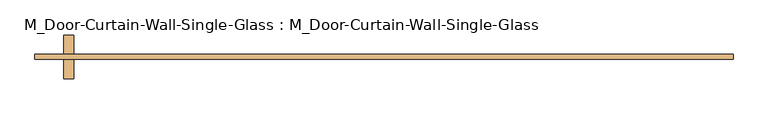
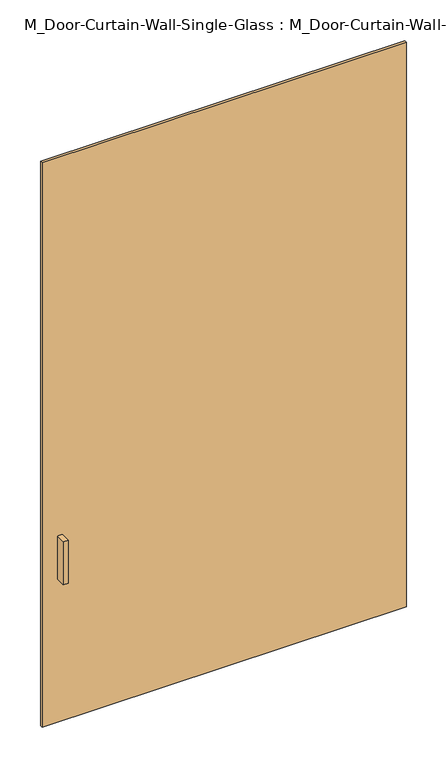
"""IFC4 building model written with IfcOpenShell, lengths in millimetres: door geometry, M_Door-Curtain-Wall-Single-Glass : M_Door-Curtain-Wall-Single-Glass."""

import ifcopenshell
import ifcopenshell.guid

model = None  # the IFC model being written
_history = None  # IfcOwnerHistory: only IFC2X3 demands one
_inside = {}  # id of a spatial element -> (the spatial element, [elements in it])
_under = {}  # id of a project, library or spatial element -> (it, [spatial elements below it])
_declared = {}  # id of a project -> (the project, [libraries it declares])
_typed = {}  # id of a type object -> (the type object, [elements of that type])
_made_of = {}  # id of a material, layer set ... -> (it, [elements and type objects made of it])


def new_model(schema):
    """Start an empty IFC model of exactly this schema.

    Asked for "IFC4X3", IfcOpenShell would pick the latest addendum, in which some entities
    have other attributes; the version numbers below select the first issue.
    IFC2X3 requires an IfcOwnerHistory on every rooted entity: one is made here for all.
    """
    global model, _history
    if schema == "IFC4X3":
        model = ifcopenshell.file(schema_version=(4, 3, 0, 0))
    else:
        model = ifcopenshell.file(schema=schema)
    _inside.clear()
    _under.clear()
    _declared.clear()
    _typed.clear()
    _made_of.clear()
    _history = None
    if model.schema == "IFC2X3":
        org = make("IfcOrganization", Name="unknown")
        user = make(
            "IfcPersonAndOrganization",
            ThePerson=make("IfcPerson", FamilyName="unknown"),
            TheOrganization=org,
        )
        app = make(
            "IfcApplication",
            ApplicationDeveloper=org,
            Version="unknown",
            ApplicationFullName="unknown",
            ApplicationIdentifier="unknown",
        )
        _history = make(
            "IfcOwnerHistory",
            OwningUser=user,
            OwningApplication=app,
            ChangeAction="ADDED",
            CreationDate=0,
        )
    return model


def make(cls, **values):
    """One entity of the class cls with the attributes given. An attribute that is None is left unset."""
    return model.create_entity(
        cls, **{name: value for name, value in values.items() if value is not None}
    )


def rooted(cls, **values):
    """An entity with a GlobalId (a new one), such as an element, a storey or a relation."""
    return make(cls, GlobalId=ifcopenshell.guid.new(), OwnerHistory=_history, **values)


def si_unit(unit_type, name, prefix=None):
    """IfcSIUnit, for example si_unit("LENGTHUNIT", "METRE", prefix="MILLI")."""
    return make("IfcSIUnit", UnitType=unit_type, Prefix=prefix, Name=name)


def assignment(units):
    """IfcUnitAssignment: the units of a project."""
    return None if units is None else make("IfcUnitAssignment", Units=units)


def point(xyz):
    """IfcCartesianPoint."""
    return None if xyz is None else make("IfcCartesianPoint", Coordinates=xyz)


def direction(xyz):
    """IfcDirection."""
    return None if xyz is None else make("IfcDirection", DirectionRatios=xyz)


def frame(location, z_axis=None, x_axis=None):
    """IfcAxis2Placement3D, a coordinate frame: its origin and axes. An axis left out is left unset."""
    return make(
        "IfcAxis2Placement3D",
        Location=point(location),
        Axis=direction(z_axis),
        RefDirection=direction(x_axis),
    )


def origin():
    """The frame at (0, 0, 0) with its axes left unset."""
    return frame((0.0, 0.0, 0.0))


def origin_with_axes():
    """The frame at (0, 0, 0) with the z axis (0, 0, 1) and the x axis (1, 0, 0) written out."""
    return frame((0.0, 0.0, 0.0), z_axis=(0.0, 0.0, 1.0), x_axis=(1.0, 0.0, 0.0))


def place(relative_to, where):
    """IfcLocalPlacement: puts the frame where relative to a parent placement (None: the world)."""
    return make(
        "IfcLocalPlacement", PlacementRelTo=relative_to, RelativePlacement=where
    )


def context(
    kind, dimensions, precision=None, world=None, true_north=None, identifier=None
):
    """IfcGeometricRepresentationContext, for example the 3D "Model" context."""
    return make(
        "IfcGeometricRepresentationContext",
        ContextIdentifier=identifier,
        ContextType=kind,
        CoordinateSpaceDimension=dimensions,
        Precision=precision,
        WorldCoordinateSystem=world,
        TrueNorth=true_north,
    )


def project(units=None, contexts=None):
    """IfcProject with its units and contexts."""
    return rooted(
        "IfcProject",
        Name="project",
        RepresentationContexts=contexts,
        UnitsInContext=assignment(units),
    )


def spatial(cls, under=None, at=None, **own):
    """A site, building, storey or space (cls), placed at a placement, below another one or the project."""
    s = rooted(cls, ObjectPlacement=at, **own)
    if under is not None:
        _under.setdefault(under.id(), (under, []))[1].append(s)
    return s


def polyline(points):
    """IfcPolyline through the points."""
    return make("IfcPolyline", Points=[point(p) for p in points])


def outline(outer, holes=None, kind="AREA"):
    """IfcArbitraryClosedProfileDef: a profile drawn as a closed curve; with holes, ...WithVoids."""
    if holes is None:
        return make("IfcArbitraryClosedProfileDef", ProfileType=kind, OuterCurve=outer)
    return make(
        "IfcArbitraryProfileDefWithVoids",
        ProfileType=kind,
        OuterCurve=outer,
        InnerCurves=holes,
    )


def extrude(swept, where, along, depth):
    """IfcExtrudedAreaSolid: the profile swept, set in the frame where, extruded along a direction by depth."""
    return make(
        "IfcExtrudedAreaSolid",
        SweptArea=swept,
        Position=where,
        ExtrudedDirection=direction(along),
        Depth=depth,
    )


def shape(context_of_items, identifier, shape_type, items):
    """IfcShapeRepresentation: the items that make up one representation, for example the "Body"."""
    return make(
        "IfcShapeRepresentation",
        ContextOfItems=context_of_items,
        RepresentationIdentifier=identifier,
        RepresentationType=shape_type,
        Items=items,
    )


def source(mapping_origin, context_of_items, identifier, shape_type, items):
    """IfcRepresentationMap: a shape defined once, which mapped items show again and again."""
    return make(
        "IfcRepresentationMap",
        MappingOrigin=mapping_origin,
        MappedRepresentation=shape(context_of_items, identifier, shape_type, items),
    )


def transform(
    local_origin,
    x_axis=None,
    y_axis=None,
    z_axis=None,
    scale=None,
    scale2=None,
    scale3=None,
    uniform=True,
):
    """IfcCartesianTransformationOperator3D, or its non-uniform kind. x_axis, y_axis, z_axis: its Axis1, 2, 3."""
    if uniform:
        return make(
            "IfcCartesianTransformationOperator3D",
            Axis1=direction(x_axis),
            Axis2=direction(y_axis),
            LocalOrigin=point(local_origin),
            Scale=scale,
            Axis3=direction(z_axis),
        )
    return make(
        "IfcCartesianTransformationOperator3DnonUniform",
        Axis1=direction(x_axis),
        Axis2=direction(y_axis),
        LocalOrigin=point(local_origin),
        Scale=scale,
        Axis3=direction(z_axis),
        Scale2=scale2,
        Scale3=scale3,
    )


def mapped(mapping_source, mapping_target):
    """IfcMappedItem: shows the shape of a source again, moved by a transform."""
    return make(
        "IfcMappedItem", MappingSource=mapping_source, MappingTarget=mapping_target
    )


def made_of(thing, what):
    """Note that an element or type object is made of a material, layer set ...; save() writes the relation."""
    if what is not None:
        _made_of.setdefault(what.id(), (what, []))[1].append(thing)
    return thing


def element(
    cls,
    number,
    at=None,
    inside=None,
    cuts=None,
    type_object=None,
    material=None,
    context=None,
    identifier="Body",
    shape_type=None,
    held_by="IfcProductDefinitionShape",
    body=None,
    shapes=None,
    **own,
):
    """One element of the class cls, such as IfcWall. Its Tag is "e" and its number.

    at: its placement. inside: the storey or other place that contains it. cuts: it is an
    opening in that element (IfcRelVoidsElement). A single representation is given by context,
    identifier, shape_type and body (its items); several are given by shapes. held_by: the class
    of the entity that holds the representations. save() writes the other relations.
    """
    e = rooted(cls, Tag="e%d" % number, ObjectPlacement=at, **own)
    if body is not None:
        shapes = [shape(context, identifier, shape_type, body)]
    if shapes is not None:
        e.Representation = make(held_by, Representations=shapes)
    if inside is not None:
        _inside.setdefault(inside.id(), (inside, []))[1].append(e)
    if cuts is not None:
        rooted(
            "IfcRelVoidsElement", RelatingBuildingElement=cuts, RelatedOpeningElement=e
        )
    if type_object is not None:
        _typed.setdefault(type_object.id(), (type_object, []))[1].append(e)
    return made_of(e, material)


def aggregate(whole, parts):
    """IfcRelAggregates: a whole, such as a stair, and the parts it consists of."""
    return rooted("IfcRelAggregates", RelatingObject=whole, RelatedObjects=parts)


def save(model, path):
    """Write the relations noted so far, then the file.

    IfcRelAggregates (storeys below a building ...), IfcRelContainedInSpatialStructure (elements
    in a storey), IfcRelDefinesByType, IfcRelAssociatesMaterial and IfcRelDeclares: one each for
    every whole, place, type object, material and project.
    """
    for whole, parts in _under.values():
        aggregate(whole, parts)
    for where, things in _inside.values():
        rooted(
            "IfcRelContainedInSpatialStructure",
            RelatedElements=things,
            RelatingStructure=where,
        )
    for kind, things in _typed.values():
        rooted("IfcRelDefinesByType", RelatedObjects=things, RelatingType=kind)
    for what, things in _made_of.values():
        rooted("IfcRelAssociatesMaterial", RelatedObjects=things, RelatingMaterial=what)
    for by, libraries in _declared.values():
        rooted("IfcRelDeclares", RelatingContext=by, RelatedDefinitions=libraries)
    model.write(path)


def m_door_curtain_wall_single_glass_m_door_curtain_wall_single_8e850fb9(model_context):
    return source(origin(), model_context, "Body", "SweptSolid", [
        extrude(outline(polyline([(916.2866169, 50.8), (916.2866169, 38.1), (-916.2866169, 38.1), (-916.2866169, 50.8), (916.2866169, 50.8)])), origin_with_axes(), (0.0, 0.0, 1.0), 3000.0),
        extrude(outline(polyline([(-814.6866169, -12.7), (-840.0866169, -12.7), (-840.0866169, 38.1), (-814.6866169, 38.1), (-814.6866169, -12.7)])), frame((0.0, 0.0, 762.0), z_axis=(0.0, 0.0, 1.0), x_axis=(1.0, 0.0, 0.0)), (0.0, 0.0, 1.0), 228.6),
        extrude(outline(polyline([(-840.0866169, 101.6), (-814.6866169, 101.6), (-814.6866169, 50.8), (-840.0866169, 50.8), (-840.0866169, 101.6)])), frame((0.0, 0.0, 762.0), z_axis=(0.0, 0.0, 1.0), x_axis=(1.0, 0.0, 0.0)), (0.0, 0.0, 1.0), 228.6),
    ])


if __name__ == "__main__":
    model = new_model("IFC4")
    model_context = context("Model", 3, world=origin())
    ifc_project = project(units=[si_unit("LENGTHUNIT", "METRE", prefix="MILLI")], contexts=[model_context])
    site = spatial("IfcSite", under=ifc_project)
    building = spatial("IfcBuilding", under=site)
    placement = place(None, origin())
    m_door_curtain_wall_single_glass_m_door_curtain_wall_single_shape = m_door_curtain_wall_single_glass_m_door_curtain_wall_single_8e850fb9(model_context)
    element("IfcDoor", 1, ObjectType="M_Door-Curtain-Wall-Single-Glass : M_Door-Curtain-Wall-Single-Glass", at=placement, inside=building, context=model_context, shape_type="MappedRepresentation", body=[
        mapped(m_door_curtain_wall_single_glass_m_door_curtain_wall_single_shape, transform((0.0, 0.0, 0.0), x_axis=(1.0, 0.0, 0.0), y_axis=(0.0, 1.0, 0.0), z_axis=(0.0, 0.0, 1.0))),
    ])
    save(model, "model.ifc")

# Revit data of these elements
# Type "M_Door-Curtain-Wall-Single-Glass : M_Door-Curtain-Wall-Single-Glass"
#   Type Mark = "23"
#   Assembly Code = "B2030100"
#   Analytic Construction = "<None>"
#   Width [instance default] = 0.9 m
#   Thermal Resistance (R) = 1.7611 (m²·K)/W
#   Swing Angle [instance default] = 90.00°
#   Heat Transfer Coefficient (U) = 0.567826 W/(m²·K)
#   Offset = 0.0508 m
#   Function = 1
#   Door Handle Material = Aluminum
#   Glazing = Glass
#   Visual Light Transmittance = 0
#   Solar Heat Gain Coefficient = 0
#   Construction Type Id = ""
# Element 1 (IfcDoor, "M_Door-Curtain-Wall-Single-Glass : M_Door-Curtain-Wall-Single-Glass")
#   Width = 1.832573 m
#   Materials on its faces: "Aluminum", "Glass"
# Materials
#   "Aluminum": class "Metal", colour RGB 244 244 244, transparency 0, Description = "Aluminum 6061", Cost = 0
#   "Glass": class "Glass", colour RGB 218 227 224, transparency 0.85, Description = "Soda Lime Glass", Cost = 0
